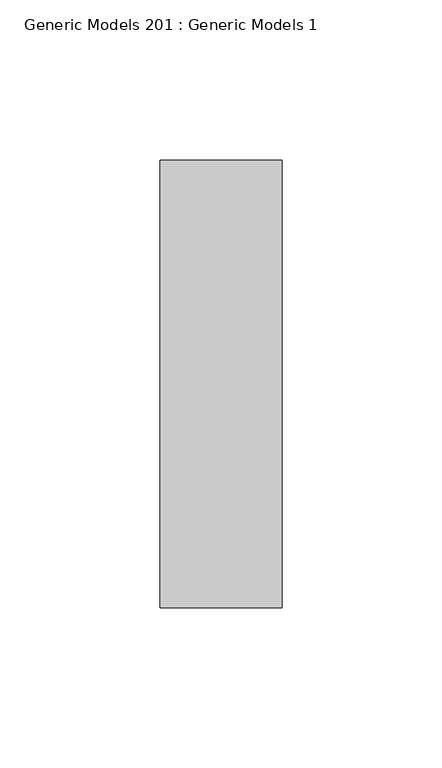
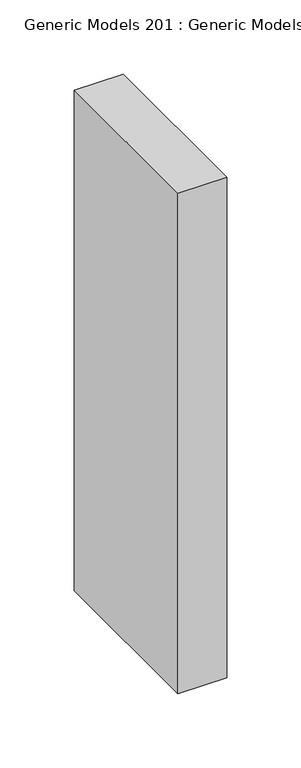
"""IFC4 building model written with IfcOpenShell, lengths in millimetres: proxy geometry, Generic Models 201 : Generic Models 1."""

import ifcopenshell
import ifcopenshell.guid

model = None  # the IFC model being written
_history = None  # IfcOwnerHistory: only IFC2X3 demands one
_inside = {}  # id of a spatial element -> (the spatial element, [elements in it])
_under = {}  # id of a project, library or spatial element -> (it, [spatial elements below it])
_declared = {}  # id of a project -> (the project, [libraries it declares])
_typed = {}  # id of a type object -> (the type object, [elements of that type])
_made_of = {}  # id of a material, layer set ... -> (it, [elements and type objects made of it])


def new_model(schema):
    """Start an empty IFC model of exactly this schema.

    Asked for "IFC4X3", IfcOpenShell would pick the latest addendum, in which some entities
    have other attributes; the version numbers below select the first issue.
    IFC2X3 requires an IfcOwnerHistory on every rooted entity: one is made here for all.
    """
    global model, _history
    if schema == "IFC4X3":
        model = ifcopenshell.file(schema_version=(4, 3, 0, 0))
    else:
        model = ifcopenshell.file(schema=schema)
    _inside.clear()
    _under.clear()
    _declared.clear()
    _typed.clear()
    _made_of.clear()
    _history = None
    if model.schema == "IFC2X3":
        org = make("IfcOrganization", Name="unknown")
        user = make(
            "IfcPersonAndOrganization",
            ThePerson=make("IfcPerson", FamilyName="unknown"),
            TheOrganization=org,
        )
        app = make(
            "IfcApplication",
            ApplicationDeveloper=org,
            Version="unknown",
            ApplicationFullName="unknown",
            ApplicationIdentifier="unknown",
        )
        _history = make(
            "IfcOwnerHistory",
            OwningUser=user,
            OwningApplication=app,
            ChangeAction="ADDED",
            CreationDate=0,
        )
    return model


def make(cls, **values):
    """One entity of the class cls with the attributes given. An attribute that is None is left unset."""
    return model.create_entity(
        cls, **{name: value for name, value in values.items() if value is not None}
    )


def rooted(cls, **values):
    """An entity with a GlobalId (a new one), such as an element, a storey or a relation."""
    return make(cls, GlobalId=ifcopenshell.guid.new(), OwnerHistory=_history, **values)


def si_unit(unit_type, name, prefix=None):
    """IfcSIUnit, for example si_unit("LENGTHUNIT", "METRE", prefix="MILLI")."""
    return make("IfcSIUnit", UnitType=unit_type, Prefix=prefix, Name=name)


def assignment(units):
    """IfcUnitAssignment: the units of a project."""
    return None if units is None else make("IfcUnitAssignment", Units=units)


def point(xyz):
    """IfcCartesianPoint."""
    return None if xyz is None else make("IfcCartesianPoint", Coordinates=xyz)


def direction(xyz):
    """IfcDirection."""
    return None if xyz is None else make("IfcDirection", DirectionRatios=xyz)


def frame(location, z_axis=None, x_axis=None):
    """IfcAxis2Placement3D, a coordinate frame: its origin and axes. An axis left out is left unset."""
    return make(
        "IfcAxis2Placement3D",
        Location=point(location),
        Axis=direction(z_axis),
        RefDirection=direction(x_axis),
    )


def origin():
    """The frame at (0, 0, 0) with its axes left unset."""
    return frame((0.0, 0.0, 0.0))


def place(relative_to, where):
    """IfcLocalPlacement: puts the frame where relative to a parent placement (None: the world)."""
    return make(
        "IfcLocalPlacement", PlacementRelTo=relative_to, RelativePlacement=where
    )


def context(
    kind, dimensions, precision=None, world=None, true_north=None, identifier=None
):
    """IfcGeometricRepresentationContext, for example the 3D "Model" context."""
    return make(
        "IfcGeometricRepresentationContext",
        ContextIdentifier=identifier,
        ContextType=kind,
        CoordinateSpaceDimension=dimensions,
        Precision=precision,
        WorldCoordinateSystem=world,
        TrueNorth=true_north,
    )


def project(units=None, contexts=None):
    """IfcProject with its units and contexts."""
    return rooted(
        "IfcProject",
        Name="project",
        RepresentationContexts=contexts,
        UnitsInContext=assignment(units),
    )


def spatial(cls, under=None, at=None, **own):
    """A site, building, storey or space (cls), placed at a placement, below another one or the project."""
    s = rooted(cls, ObjectPlacement=at, **own)
    if under is not None:
        _under.setdefault(under.id(), (under, []))[1].append(s)
    return s


def polyline(points):
    """IfcPolyline through the points."""
    return make("IfcPolyline", Points=[point(p) for p in points])


def outline(outer, holes=None, kind="AREA"):
    """IfcArbitraryClosedProfileDef: a profile drawn as a closed curve; with holes, ...WithVoids."""
    if holes is None:
        return make("IfcArbitraryClosedProfileDef", ProfileType=kind, OuterCurve=outer)
    return make(
        "IfcArbitraryProfileDefWithVoids",
        ProfileType=kind,
        OuterCurve=outer,
        InnerCurves=holes,
    )


def extrude(swept, where, along, depth):
    """IfcExtrudedAreaSolid: the profile swept, set in the frame where, extruded along a direction by depth."""
    return make(
        "IfcExtrudedAreaSolid",
        SweptArea=swept,
        Position=where,
        ExtrudedDirection=direction(along),
        Depth=depth,
    )


def shape(context_of_items, identifier, shape_type, items):
    """IfcShapeRepresentation: the items that make up one representation, for example the "Body"."""
    return make(
        "IfcShapeRepresentation",
        ContextOfItems=context_of_items,
        RepresentationIdentifier=identifier,
        RepresentationType=shape_type,
        Items=items,
    )


def source(mapping_origin, context_of_items, identifier, shape_type, items):
    """IfcRepresentationMap: a shape defined once, which mapped items show again and again."""
    return make(
        "IfcRepresentationMap",
        MappingOrigin=mapping_origin,
        MappedRepresentation=shape(context_of_items, identifier, shape_type, items),
    )


def transform(
    local_origin,
    x_axis=None,
    y_axis=None,
    z_axis=None,
    scale=None,
    scale2=None,
    scale3=None,
    uniform=True,
):
    """IfcCartesianTransformationOperator3D, or its non-uniform kind. x_axis, y_axis, z_axis: its Axis1, 2, 3."""
    if uniform:
        return make(
            "IfcCartesianTransformationOperator3D",
            Axis1=direction(x_axis),
            Axis2=direction(y_axis),
            LocalOrigin=point(local_origin),
            Scale=scale,
            Axis3=direction(z_axis),
        )
    return make(
        "IfcCartesianTransformationOperator3DnonUniform",
        Axis1=direction(x_axis),
        Axis2=direction(y_axis),
        LocalOrigin=point(local_origin),
        Scale=scale,
        Axis3=direction(z_axis),
        Scale2=scale2,
        Scale3=scale3,
    )


def mapped(mapping_source, mapping_target):
    """IfcMappedItem: shows the shape of a source again, moved by a transform."""
    return make(
        "IfcMappedItem", MappingSource=mapping_source, MappingTarget=mapping_target
    )


def made_of(thing, what):
    """Note that an element or type object is made of a material, layer set ...; save() writes the relation."""
    if what is not None:
        _made_of.setdefault(what.id(), (what, []))[1].append(thing)
    return thing


def element(
    cls,
    number,
    at=None,
    inside=None,
    cuts=None,
    type_object=None,
    material=None,
    context=None,
    identifier="Body",
    shape_type=None,
    held_by="IfcProductDefinitionShape",
    body=None,
    shapes=None,
    **own,
):
    """One element of the class cls, such as IfcWall. Its Tag is "e" and its number.

    at: its placement. inside: the storey or other place that contains it. cuts: it is an
    opening in that element (IfcRelVoidsElement). A single representation is given by context,
    identifier, shape_type and body (its items); several are given by shapes. held_by: the class
    of the entity that holds the representations. save() writes the other relations.
    """
    e = rooted(cls, Tag="e%d" % number, ObjectPlacement=at, **own)
    if body is not None:
        shapes = [shape(context, identifier, shape_type, body)]
    if shapes is not None:
        e.Representation = make(held_by, Representations=shapes)
    if inside is not None:
        _inside.setdefault(inside.id(), (inside, []))[1].append(e)
    if cuts is not None:
        rooted(
            "IfcRelVoidsElement", RelatingBuildingElement=cuts, RelatedOpeningElement=e
        )
    if type_object is not None:
        _typed.setdefault(type_object.id(), (type_object, []))[1].append(e)
    return made_of(e, material)


def aggregate(whole, parts):
    """IfcRelAggregates: a whole, such as a stair, and the parts it consists of."""
    return rooted("IfcRelAggregates", RelatingObject=whole, RelatedObjects=parts)


def save(model, path):
    """Write the relations noted so far, then the file.

    IfcRelAggregates (storeys below a building ...), IfcRelContainedInSpatialStructure (elements
    in a storey), IfcRelDefinesByType, IfcRelAssociatesMaterial and IfcRelDeclares: one each for
    every whole, place, type object, material and project.
    """
    for whole, parts in _under.values():
        aggregate(whole, parts)
    for where, things in _inside.values():
        rooted(
            "IfcRelContainedInSpatialStructure",
            RelatedElements=things,
            RelatingStructure=where,
        )
    for kind, things in _typed.values():
        rooted("IfcRelDefinesByType", RelatedObjects=things, RelatingType=kind)
    for what, things in _made_of.values():
        rooted("IfcRelAssociatesMaterial", RelatedObjects=things, RelatingMaterial=what)
    for by, libraries in _declared.values():
        rooted("IfcRelDeclares", RelatingContext=by, RelatedDefinitions=libraries)
    model.write(path)


def generic_models_201_generic_models_1_a61de597(model_context):
    return source(origin(), model_context, "Body", "SweptSolid", [
        extrude(outline(polyline([(-2894.120657, -5448.3625551), (-2932.220657, -5448.3625551), (-2932.220657, -5308.6625551), (-2894.120657, -5308.6625551), (-2894.120657, -5448.3625551)])), frame((0.0, 0.0, 126821.946), z_axis=(0.0, 0.0, 1.0), x_axis=(1.0, 0.0, 0.0)), (0.0, 0.0, 1.0), 412.2820113),
    ])


if __name__ == "__main__":
    model = new_model("IFC4")
    model_context = context("Model", 3, world=origin())
    ifc_project = project(units=[si_unit("LENGTHUNIT", "METRE", prefix="MILLI")], contexts=[model_context])
    site = spatial("IfcSite", under=ifc_project)
    building = spatial("IfcBuilding", under=site)
    placement = place(None, origin())
    generic_models_201_generic_models_1_shape = generic_models_201_generic_models_1_a61de597(model_context)
    element("IfcBuildingElementProxy", 1, Name="Generic Models 201 : Generic Models 1", ObjectType="Generic Models 201 : Generic Models 1", at=placement, inside=building, context=model_context, shape_type="MappedRepresentation", body=[
        mapped(generic_models_201_generic_models_1_shape, transform((0.0, 0.0, 0.0), x_axis=(1.0, 0.0, 0.0), y_axis=(0.0, 1.0, 0.0), z_axis=(0.0, 0.0, 1.0))),
    ])
    save(model, "model.ifc")

# Revit data of these elements
# Element 1 (IfcBuildingElementProxy, "Generic Models 201 : Generic Models 1")
#   Materials on its faces: "_2X BLOCKING AS REQUIRED"
# Materials
#   "_2X BLOCKING AS REQUIRED": class "Generic", colour RGB 177 130 114, transparency 0, Cost = 0
